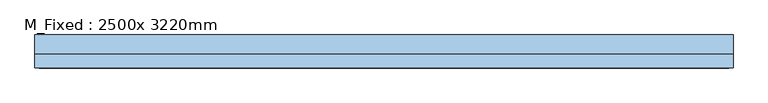
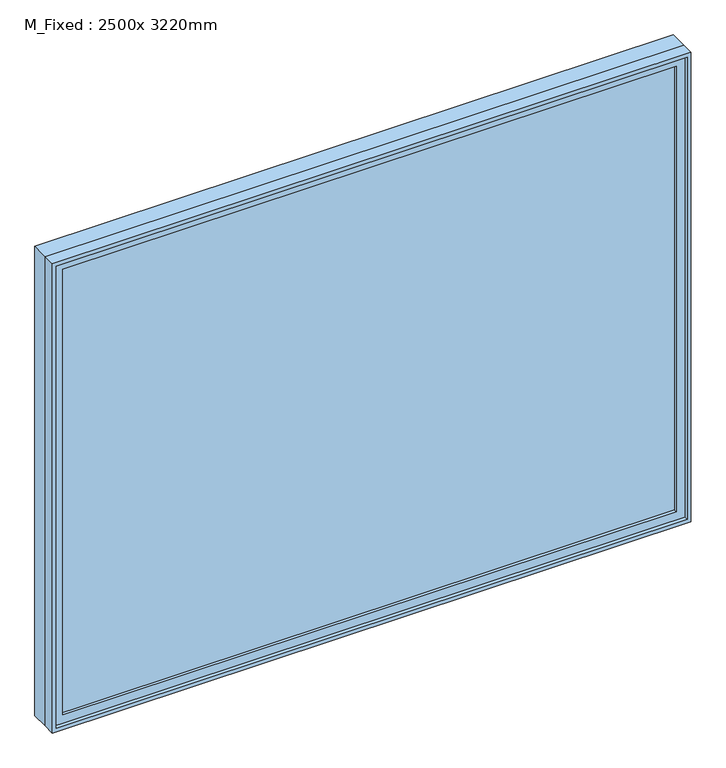
"""IFC4 building model written with IfcOpenShell, lengths in millimetres: window geometry, M_Fixed : 2500x 3220mm."""

from ifc_helpers import new_model, si_unit, frame, origin, place, context, project, spatial, polyline, outline, extrude, source, transform, mapped, element, save


def m_fixed_2500x_3220mm_8b997f8c(model_context):
    return source(origin(), model_context, "Body", "SweptSolid", [
        extrude(outline(polyline([(-1546.8, -54.2), (-1546.8, -42.2), (1546.8, -42.2), (1546.8, -54.2), (-1546.8, -54.2)])), frame((0.0, 0.0, 368.0), z_axis=(0.0, 0.0, 1.0), x_axis=(1.0, 0.0, 0.0)), (0.0, 0.0, 1.0), 2374.0),
        extrude(outline(polyline([(2786.0, -1590.8), (324.0, -1590.8), (324.0, 1590.8), (2786.0, 1590.8), (2786.0, -1590.8)]), holes=[polyline([(2742.0, -1546.8), (2742.0, 1546.8), (368.0, 1546.8), (368.0, -1546.8), (2742.0, -1546.8)])]), frame((0.0, -70.2, 0.0), z_axis=(0.0, 1.0, 0.0), x_axis=(0.0, 0.0, 1.0)), (0.0, 0.0, 1.0), 44.0),
        extrude(outline(polyline([(2805.0, -1609.8), (305.0, -1609.8), (305.0, 1609.8), (2805.0, 1609.8), (2805.0, -1609.8)]), holes=[polyline([(2786.0, -1590.8), (2786.0, 1590.8), (324.0, 1590.8), (324.0, -1590.8), (2786.0, -1590.8)])]), frame((0.0, -89.2, 0.0), z_axis=(0.0, 1.0, 0.0), x_axis=(0.0, 0.0, 1.0)), (0.0, 0.0, 1.0), 63.0),
        extrude(outline(polyline([(2805.0, -1609.8), (305.0, -1609.8), (305.0, 1609.8), (2805.0, 1609.8), (2805.0, -1609.8)]), holes=[polyline([(2773.0, -1577.8), (2773.0, 1577.8), (337.0, 1577.8), (337.0, -1577.8), (2773.0, -1577.8)])]), frame((0.0, -26.2, 0.0), z_axis=(0.0, 1.0, 0.0), x_axis=(0.0, 0.0, 1.0)), (0.0, 0.0, 1.0), 89.4),
    ])


if __name__ == "__main__":
    model = new_model("IFC4")
    model_context = context("Model", 3, world=origin())
    ifc_project = project(units=[si_unit("LENGTHUNIT", "METRE", prefix="MILLI")], contexts=[model_context])
    site = spatial("IfcSite", under=ifc_project)
    building = spatial("IfcBuilding", under=site)
    placement = place(None, origin())
    m_fixed_2500x_3220mm_shape = m_fixed_2500x_3220mm_8b997f8c(model_context)
    element("IfcWindow", 1, ObjectType="M_Fixed : 2500x 3220mm", at=placement, inside=building, context=model_context, shape_type="MappedRepresentation", body=[
        mapped(m_fixed_2500x_3220mm_shape, transform((0.0, 0.0, 0.0), x_axis=(1.0, 0.0, 0.0), y_axis=(0.0, 1.0, 0.0), z_axis=(0.0, 0.0, 1.0))),
    ])
    save(model, "model.ifc")

# Revit data of these elements
# Type "M_Fixed : 2500x 3220mm"
#   Type Mark = "26"
#   Height = 2500 mm
#   Default Sill Height = 305 mm
#   Width = 3219.6 mm
#   Window Inset = 19 mm
#   Frame Exterior Material = Sash
#   Frame Interior Material = Sash
#   Glass Pane Material = Glass
#   Sash = Sash
#   Wall Closure = (empty or 0)
# Element 1 (IfcWindow, "M_Fixed : 2500x 3220mm")
#   Materials on its faces: "Sash", "Glass"
# Materials
#   "Sash": class "Wood", colour RGB 136 99 55, transparency 0
#   "Glass": class "Glass", colour RGB 0 128 192, transparency 0.9, Description = "Soda Lime Glass", Cost = 0
